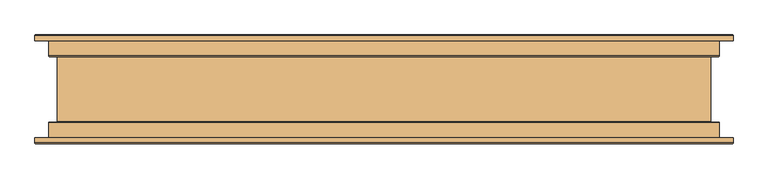
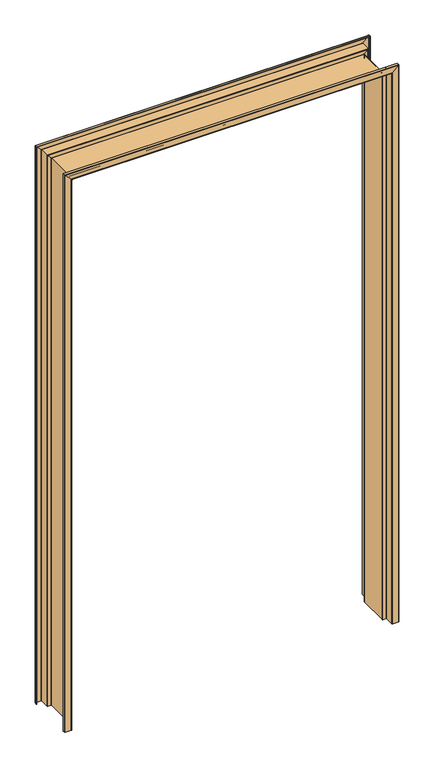
"""IFC4 building model written with IfcOpenShell, lengths in millimetres: door geometry, Porta Dupla de Abrir : 120x210cm - Marco Metálico."""

from ifc_helpers import new_model, si_unit, frame, origin, place, context, project, spatial, polyline, circle_curve, ellipse_curve, source, transform, mapped, element, save
from ifc_brep_helpers import plane_surface, cylinder_surface, revolved_surface, advanced_brep


def door_964c49d4(model_context):
    return source(origin(), model_context, "Body", "AdvancedBrep", [
        advanced_brep(
        [(-574.05, 57.1, 50.0), (-574.05, -57.1, 50.0), (-575.55, -58.6, 50.0), (-588.55, -58.6, 50.0), (-589.05, -59.1, 50.0), (-589.05, -94.1, 50.0), (-590.55, -95.6, 50.0), (-612.55, -95.6, 50.0), (-614.05, -94.1, 50.0), (-614.05, -85.6, 50.0), (-613.05, -85.6, 50.0), (-613.05, -94.1, 50.0), (-612.55, -94.6, 50.0), (-590.55, -94.6, 50.0), (-590.05, -94.1, 50.0), (-590.05, -59.1, 50.0), (-588.55, -57.6, 50.0), (-575.55, -57.6, 50.0), (-575.05, -57.1, 50.0), (-575.05, 57.1, 50.0), (-575.55, 57.6, 50.0), (-588.55, 57.6, 50.0), (-590.05, 59.1, 50.0), (-590.05, 94.1, 50.0), (-590.55, 94.6, 50.0), (-612.55, 94.6, 50.0), (-613.05, 94.1, 50.0), (-613.05, 85.6, 50.0), (-614.05, 85.6, 50.0), (-614.05, 94.1, 50.0), (-612.55, 95.6, 50.0), (-590.55, 95.6, 50.0), (-589.05, 94.1, 50.0), (-589.05, 59.1, 50.0), (-588.55, 58.6, 50.0), (-575.55, 58.6, 50.0), (-574.05, 57.1, 2174.05), (-574.05, -57.1, 2174.05), (-575.55, -58.6, 2175.55), (-588.55, -58.6, 2188.55), (-589.05, -59.1, 2189.05), (-589.05, -94.1, 2189.05), (-590.55, -95.6, 2190.55), (-612.55, -95.6, 2212.55), (-614.05, -94.1, 2214.05), (-614.05, -85.6, 2214.05), (-613.05, -85.6, 2213.05), (-613.05, -94.1, 2213.05), (-612.55, -94.6, 2212.55), (-590.55, -94.6, 2190.55), (-590.05, -94.1, 2190.05), (-590.05, -59.1, 2190.05), (-588.55, -57.6, 2188.55), (-575.55, -57.6, 2175.55), (-575.05, -57.1, 2175.05), (-575.05, 57.1, 2175.05), (-575.55, 57.6, 2175.55), (-588.55, 57.6, 2188.55), (-590.05, 59.1, 2190.05), (-590.05, 94.1, 2190.05), (-590.55, 94.6, 2190.55), (-612.55, 94.6, 2212.55), (-613.05, 94.1, 2213.05), (-613.05, 85.6, 2213.05), (-614.05, 85.6, 2214.05), (-614.05, 94.1, 2214.05), (-612.55, 95.6, 2212.55), (-590.55, 95.6, 2190.55), (-589.05, 94.1, 2189.05), (-589.05, 59.1, 2189.05), (-588.55, 58.6, 2188.55), (-575.55, 58.6, 2175.55), (574.05, 57.1, 50.0), (575.55, 58.6, 50.0), (588.55, 58.6, 50.0), (589.05, 59.1, 50.0), (589.05, 94.1, 50.0), (590.55, 95.6, 50.0), (612.55, 95.6, 50.0), (614.05, 94.1, 50.0), (614.05, 85.6, 50.0), (613.05, 85.6, 50.0), (613.05, 94.1, 50.0), (612.55, 94.6, 50.0), (590.55, 94.6, 50.0), (590.05, 94.1, 50.0), (590.05, 59.1, 50.0), (588.55, 57.6, 50.0), (575.55, 57.6, 50.0), (575.05, 57.1, 50.0), (575.05, -57.1, 50.0), (575.55, -57.6, 50.0), (588.55, -57.6, 50.0), (590.05, -59.1, 50.0), (590.05, -94.1, 50.0), (590.55, -94.6, 50.0), (612.55, -94.6, 50.0), (613.05, -94.1, 50.0), (613.05, -85.6, 50.0), (614.05, -85.6, 50.0), (614.05, -94.1, 50.0), (612.55, -95.6, 50.0), (590.55, -95.6, 50.0), (589.05, -94.1, 50.0), (589.05, -59.1, 50.0), (588.55, -58.6, 50.0), (575.55, -58.6, 50.0), (574.05, -57.1, 50.0), (574.05, 57.1, 2174.05), (575.55, 58.6, 2175.55), (588.55, 58.6, 2188.55), (589.05, 59.1, 2189.05), (589.05, 94.1, 2189.05), (590.55, 95.6, 2190.55), (612.55, 95.6, 2212.55), (614.05, 94.1, 2214.05), (614.05, 85.6, 2214.05), (613.05, 85.6, 2213.05), (613.05, 94.1, 2213.05), (612.55, 94.6, 2212.55), (590.55, 94.6, 2190.55), (590.05, 94.1, 2190.05), (590.05, 59.1, 2190.05), (588.55, 57.6, 2188.55), (575.55, 57.6, 2175.55), (575.05, 57.1, 2175.05), (575.05, -57.1, 2175.05), (575.55, -57.6, 2175.55), (588.55, -57.6, 2188.55), (590.05, -59.1, 2190.05), (590.05, -94.1, 2190.05), (590.55, -94.6, 2190.55), (612.55, -94.6, 2212.55), (613.05, -94.1, 2213.05), (613.05, -85.6, 2213.05), (614.05, -85.6, 2214.05), (614.05, -94.1, 2214.05), (612.55, -95.6, 2212.55), (590.55, -95.6, 2190.55), (589.05, -94.1, 2189.05), (589.05, -59.1, 2189.05), (588.55, -58.6, 2188.55), (575.55, -58.6, 2175.55), (574.05, -57.1, 2174.05)],
        [
            (0, 1),
            (1, 2, circle_curve(frame((-575.55, -57.1, 50.0), z_axis=(0.0, 0.0, -1.0), x_axis=(1.0, 0.0, 0.0)), 1.5)),
            (2, 3),
            (3, 4, circle_curve(frame((-588.55, -59.1, 50.0), z_axis=(0.0, 0.0, 1.0), x_axis=(1.0, 0.0, 0.0)), 0.5)),
            (4, 5),
            (5, 6, circle_curve(frame((-590.55, -94.1, 50.0), z_axis=(0.0, 0.0, -1.0), x_axis=(1.0, 0.0, 0.0)), 1.5)),
            (6, 7),
            (7, 8, circle_curve(frame((-612.55, -94.1, 50.0), z_axis=(0.0, 0.0, -1.0), x_axis=(1.0, 0.0, 0.0)), 1.5)),
            (8, 9),
            (9, 10),
            (10, 11),
            (11, 12, circle_curve(frame((-612.55, -94.1, 50.0), z_axis=(0.0, 0.0, 1.0), x_axis=(1.0, 0.0, 0.0)), 0.5)),
            (12, 13),
            (13, 14, circle_curve(frame((-590.55, -94.1, 50.0), z_axis=(0.0, 0.0, 1.0), x_axis=(1.0, 0.0, 0.0)), 0.5)),
            (14, 15),
            (15, 16, circle_curve(frame((-588.55, -59.1, 50.0), z_axis=(0.0, 0.0, -1.0), x_axis=(1.0, 0.0, 0.0)), 1.5)),
            (16, 17),
            (17, 18, circle_curve(frame((-575.55, -57.1, 50.0), z_axis=(0.0, 0.0, 1.0), x_axis=(1.0, 0.0, 0.0)), 0.5)),
            (18, 19),
            (19, 20, circle_curve(frame((-575.55, 57.1, 50.0), z_axis=(0.0, 0.0, 1.0), x_axis=(1.0, 0.0, 0.0)), 0.5)),
            (20, 21),
            (21, 22, circle_curve(frame((-588.55, 59.1, 50.0), z_axis=(0.0, 0.0, -1.0), x_axis=(1.0, 0.0, 0.0)), 1.5)),
            (22, 23),
            (23, 24, circle_curve(frame((-590.55, 94.1, 50.0), z_axis=(0.0, 0.0, 1.0), x_axis=(1.0, 0.0, 0.0)), 0.5)),
            (24, 25),
            (25, 26, circle_curve(frame((-612.55, 94.1, 50.0), z_axis=(0.0, 0.0, 1.0), x_axis=(1.0, 0.0, 0.0)), 0.5)),
            (26, 27),
            (27, 28),
            (28, 29),
            (29, 30, circle_curve(frame((-612.55, 94.1, 50.0), z_axis=(0.0, 0.0, -1.0), x_axis=(1.0, 0.0, 0.0)), 1.5)),
            (30, 31),
            (31, 32, circle_curve(frame((-590.55, 94.1, 50.0), z_axis=(0.0, 0.0, -1.0), x_axis=(1.0, 0.0, 0.0)), 1.5)),
            (32, 33),
            (33, 34, circle_curve(frame((-588.55, 59.1, 50.0), z_axis=(0.0, 0.0, 1.0), x_axis=(1.0, 0.0, 0.0)), 0.5)),
            (34, 35),
            (35, 0, circle_curve(frame((-575.55, 57.1, 50.0), z_axis=(0.0, 0.0, -1.0), x_axis=(1.0, 0.0, 0.0)), 1.5)),
            (0, 36),
            (36, 37),
            (37, 1),
            (37, 38, ellipse_curve(frame((-575.55, -57.1, 2175.55), z_axis=(-0.7071067811865475, 0.0, -0.7071067811865475), x_axis=(0.7071067811865474, 0.0, -0.7071067811865476)), 2.1213203, 1.5)),
            (38, 2),
            (38, 39),
            (39, 3),
            (39, 40, ellipse_curve(frame((-588.55, -59.1, 2188.55), z_axis=(0.7071067811865475, 0.0, 0.7071067811865475), x_axis=(-0.7071067811865474, 0.0, 0.7071067811865476)), 0.7071068, 0.5)),
            (40, 4),
            (40, 41),
            (41, 5),
            (41, 42, ellipse_curve(frame((-590.55, -94.1, 2190.55), z_axis=(-0.7071067811865475, 0.0, -0.7071067811865475), x_axis=(0.7071067811865474, 0.0, -0.7071067811865476)), 2.1213203, 1.5)),
            (42, 6),
            (42, 43),
            (43, 7),
            (43, 44, ellipse_curve(frame((-612.55, -94.1, 2212.55), z_axis=(-0.7071067811865475, 0.0, -0.7071067811865475), x_axis=(0.7071067811865474, 0.0, -0.7071067811865476)), 2.1213203, 1.5)),
            (44, 8),
            (44, 45),
            (45, 9),
            (45, 46),
            (46, 10),
            (46, 47),
            (47, 11),
            (47, 48, ellipse_curve(frame((-612.55, -94.1, 2212.55), z_axis=(0.7071067811865475, 0.0, 0.7071067811865475), x_axis=(-0.7071067811865474, 0.0, 0.7071067811865476)), 0.7071068, 0.5)),
            (48, 12),
            (48, 49),
            (49, 13),
            (49, 50, ellipse_curve(frame((-590.55, -94.1, 2190.55), z_axis=(0.7071067811865475, 0.0, 0.7071067811865475), x_axis=(-0.7071067811865474, 0.0, 0.7071067811865476)), 0.7071068, 0.5)),
            (50, 14),
            (50, 51),
            (51, 15),
            (51, 52, ellipse_curve(frame((-588.55, -59.1, 2188.55), z_axis=(-0.7071067811865475, 0.0, -0.7071067811865475), x_axis=(0.7071067811865474, 0.0, -0.7071067811865476)), 2.1213203, 1.5)),
            (52, 16),
            (52, 53),
            (53, 17),
            (53, 54, ellipse_curve(frame((-575.55, -57.1, 2175.55), z_axis=(0.7071067811865475, 0.0, 0.7071067811865475), x_axis=(-0.7071067811865474, 0.0, 0.7071067811865476)), 0.7071068, 0.5)),
            (54, 18),
            (54, 55),
            (55, 19),
            (55, 56, ellipse_curve(frame((-575.55, 57.1, 2175.55), z_axis=(0.7071067811865475, 0.0, 0.7071067811865475), x_axis=(-0.7071067811865474, 0.0, 0.7071067811865476)), 0.7071068, 0.5)),
            (56, 20),
            (56, 57),
            (57, 21),
            (57, 58, ellipse_curve(frame((-588.55, 59.1, 2188.55), z_axis=(-0.7071067811865475, 0.0, -0.7071067811865475), x_axis=(0.7071067811865474, 0.0, -0.7071067811865476)), 2.1213203, 1.5)),
            (58, 22),
            (58, 59),
            (59, 23),
            (59, 60, ellipse_curve(frame((-590.55, 94.1, 2190.55), z_axis=(0.7071067811865475, 0.0, 0.7071067811865475), x_axis=(-0.7071067811865474, 0.0, 0.7071067811865476)), 0.7071068, 0.5)),
            (60, 24),
            (60, 61),
            (61, 25),
            (61, 62, ellipse_curve(frame((-612.55, 94.1, 2212.55), z_axis=(0.7071067811865475, 0.0, 0.7071067811865475), x_axis=(-0.7071067811865474, 0.0, 0.7071067811865476)), 0.7071068, 0.5)),
            (62, 26),
            (62, 63),
            (63, 27),
            (63, 64),
            (64, 28),
            (64, 65),
            (65, 29),
            (65, 66, ellipse_curve(frame((-612.55, 94.1, 2212.55), z_axis=(-0.7071067811865475, 0.0, -0.7071067811865475), x_axis=(0.7071067811865474, 0.0, -0.7071067811865476)), 2.1213203, 1.5)),
            (66, 30),
            (66, 67),
            (67, 31),
            (67, 68, ellipse_curve(frame((-590.55, 94.1, 2190.55), z_axis=(-0.7071067811865475, 0.0, -0.7071067811865475), x_axis=(0.7071067811865474, 0.0, -0.7071067811865476)), 2.1213203, 1.5)),
            (68, 32),
            (68, 69),
            (69, 33),
            (69, 70, ellipse_curve(frame((-588.55, 59.1, 2188.55), z_axis=(0.7071067811865475, 0.0, 0.7071067811865475), x_axis=(-0.7071067811865474, 0.0, 0.7071067811865476)), 0.7071068, 0.5)),
            (70, 34),
            (70, 71),
            (71, 35),
            (71, 36, ellipse_curve(frame((-575.55, 57.1, 2175.55), z_axis=(-0.7071067811865475, 0.0, -0.7071067811865475), x_axis=(0.7071067811865474, 0.0, -0.7071067811865476)), 2.1213203, 1.5)),
            (72, 73, circle_curve(frame((575.55, 57.1, 50.0), z_axis=(0.0, 0.0, -1.0), x_axis=(-1.0, 0.0, 0.0)), 1.5)),
            (73, 74),
            (74, 75, circle_curve(frame((588.55, 59.1, 50.0), z_axis=(0.0, 0.0, 1.0), x_axis=(-1.0, 0.0, 0.0)), 0.5)),
            (75, 76),
            (76, 77, circle_curve(frame((590.55, 94.1, 50.0), z_axis=(0.0, 0.0, -1.0), x_axis=(-1.0, 0.0, 0.0)), 1.5)),
            (77, 78),
            (78, 79, circle_curve(frame((612.55, 94.1, 50.0), z_axis=(0.0, 0.0, -1.0), x_axis=(-1.0, 0.0, 0.0)), 1.5)),
            (79, 80),
            (80, 81),
            (81, 82),
            (82, 83, circle_curve(frame((612.55, 94.1, 50.0), z_axis=(0.0, 0.0, 1.0), x_axis=(-1.0, 0.0, 0.0)), 0.5)),
            (83, 84),
            (84, 85, circle_curve(frame((590.55, 94.1, 50.0), z_axis=(0.0, 0.0, 1.0), x_axis=(-1.0, 0.0, 0.0)), 0.5)),
            (85, 86),
            (86, 87, circle_curve(frame((588.55, 59.1, 50.0), z_axis=(0.0, 0.0, -1.0), x_axis=(-1.0, 0.0, 0.0)), 1.5)),
            (87, 88),
            (88, 89, circle_curve(frame((575.55, 57.1, 50.0), z_axis=(0.0, 0.0, 1.0), x_axis=(-1.0, 0.0, 0.0)), 0.5)),
            (89, 90),
            (90, 91, circle_curve(frame((575.55, -57.1, 50.0), z_axis=(0.0, 0.0, 1.0), x_axis=(-1.0, 0.0, 0.0)), 0.5)),
            (91, 92),
            (92, 93, circle_curve(frame((588.55, -59.1, 50.0), z_axis=(0.0, 0.0, -1.0), x_axis=(-1.0, 0.0, 0.0)), 1.5)),
            (93, 94),
            (94, 95, circle_curve(frame((590.55, -94.1, 50.0), z_axis=(0.0, 0.0, 1.0), x_axis=(-1.0, 0.0, 0.0)), 0.5)),
            (95, 96),
            (96, 97, circle_curve(frame((612.55, -94.1, 50.0), z_axis=(0.0, 0.0, 1.0), x_axis=(-1.0, 0.0, 0.0)), 0.5)),
            (97, 98),
            (98, 99),
            (99, 100),
            (100, 101, circle_curve(frame((612.55, -94.1, 50.0), z_axis=(0.0, 0.0, -1.0), x_axis=(-1.0, 0.0, 0.0)), 1.5)),
            (101, 102),
            (102, 103, circle_curve(frame((590.55, -94.1, 50.0), z_axis=(0.0, 0.0, -1.0), x_axis=(-1.0, 0.0, 0.0)), 1.5)),
            (103, 104),
            (104, 105, circle_curve(frame((588.55, -59.1, 50.0), z_axis=(0.0, 0.0, 1.0), x_axis=(-1.0, 0.0, 0.0)), 0.5)),
            (105, 106),
            (106, 107, circle_curve(frame((575.55, -57.1, 50.0), z_axis=(0.0, 0.0, -1.0), x_axis=(-1.0, 0.0, 0.0)), 1.5)),
            (107, 72),
            (108, 109, ellipse_curve(frame((575.55, 57.1, 2175.55), z_axis=(0.7071067811865475, 0.0, -0.7071067811865475), x_axis=(0.7071067811865474, 0.0, 0.7071067811865476)), 2.1213203, 1.5)),
            (109, 73),
            (72, 108),
            (109, 110),
            (110, 74),
            (110, 111, ellipse_curve(frame((588.55, 59.1, 2188.55), z_axis=(-0.7071067811865475, 0.0, 0.7071067811865475), x_axis=(-0.7071067811865474, 0.0, -0.7071067811865476)), 0.7071068, 0.5)),
            (111, 75),
            (111, 112),
            (112, 76),
            (112, 113, ellipse_curve(frame((590.55, 94.1, 2190.55), z_axis=(0.7071067811865475, 0.0, -0.7071067811865475), x_axis=(0.7071067811865474, 0.0, 0.7071067811865476)), 2.1213203, 1.5)),
            (113, 77),
            (113, 114),
            (114, 78),
            (114, 115, ellipse_curve(frame((612.55, 94.1, 2212.55), z_axis=(0.7071067811865475, 0.0, -0.7071067811865475), x_axis=(0.7071067811865474, 0.0, 0.7071067811865476)), 2.1213203, 1.5)),
            (115, 79),
            (115, 116),
            (116, 80),
            (116, 117),
            (117, 81),
            (117, 118),
            (118, 82),
            (118, 119, ellipse_curve(frame((612.55, 94.1, 2212.55), z_axis=(-0.7071067811865475, 0.0, 0.7071067811865475), x_axis=(-0.7071067811865474, 0.0, -0.7071067811865476)), 0.7071068, 0.5)),
            (119, 83),
            (119, 120),
            (120, 84),
            (120, 121, ellipse_curve(frame((590.55, 94.1, 2190.55), z_axis=(-0.7071067811865475, 0.0, 0.7071067811865475), x_axis=(-0.7071067811865474, 0.0, -0.7071067811865476)), 0.7071068, 0.5)),
            (121, 85),
            (121, 122),
            (122, 86),
            (122, 123, ellipse_curve(frame((588.55, 59.1, 2188.55), z_axis=(0.7071067811865475, 0.0, -0.7071067811865475), x_axis=(0.7071067811865474, 0.0, 0.7071067811865476)), 2.1213203, 1.5)),
            (123, 87),
            (123, 124),
            (124, 88),
            (124, 125, ellipse_curve(frame((575.55, 57.1, 2175.55), z_axis=(-0.7071067811865475, 0.0, 0.7071067811865475), x_axis=(-0.7071067811865474, 0.0, -0.7071067811865476)), 0.7071068, 0.5)),
            (125, 89),
            (125, 126),
            (126, 90),
            (126, 127, ellipse_curve(frame((575.55, -57.1, 2175.55), z_axis=(-0.7071067811865475, 0.0, 0.7071067811865475), x_axis=(-0.7071067811865474, 0.0, -0.7071067811865476)), 0.7071068, 0.5)),
            (127, 91),
            (127, 128),
            (128, 92),
            (128, 129, ellipse_curve(frame((588.55, -59.1, 2188.55), z_axis=(0.7071067811865475, 0.0, -0.7071067811865475), x_axis=(0.7071067811865474, 0.0, 0.7071067811865476)), 2.1213203, 1.5)),
            (129, 93),
            (129, 130),
            (130, 94),
            (130, 131, ellipse_curve(frame((590.55, -94.1, 2190.55), z_axis=(-0.7071067811865475, 0.0, 0.7071067811865475), x_axis=(-0.7071067811865474, 0.0, -0.7071067811865476)), 0.7071068, 0.5)),
            (131, 95),
            (131, 132),
            (132, 96),
            (132, 133, ellipse_curve(frame((612.55, -94.1, 2212.55), z_axis=(-0.7071067811865475, 0.0, 0.7071067811865475), x_axis=(-0.7071067811865474, 0.0, -0.7071067811865476)), 0.7071068, 0.5)),
            (133, 97),
            (133, 134),
            (134, 98),
            (134, 135),
            (135, 99),
            (135, 136),
            (136, 100),
            (136, 137, ellipse_curve(frame((612.55, -94.1, 2212.55), z_axis=(0.7071067811865475, 0.0, -0.7071067811865475), x_axis=(0.7071067811865474, 0.0, 0.7071067811865476)), 2.1213203, 1.5)),
            (137, 101),
            (137, 138),
            (138, 102),
            (138, 139, ellipse_curve(frame((590.55, -94.1, 2190.55), z_axis=(0.7071067811865475, 0.0, -0.7071067811865475), x_axis=(0.7071067811865474, 0.0, 0.7071067811865476)), 2.1213203, 1.5)),
            (139, 103),
            (139, 140),
            (140, 104),
            (140, 141, ellipse_curve(frame((588.55, -59.1, 2188.55), z_axis=(-0.7071067811865475, 0.0, 0.7071067811865475), x_axis=(-0.7071067811865474, 0.0, -0.7071067811865476)), 0.7071068, 0.5)),
            (141, 105),
            (141, 142),
            (142, 106),
            (142, 143, ellipse_curve(frame((575.55, -57.1, 2175.55), z_axis=(0.7071067811865475, 0.0, -0.7071067811865475), x_axis=(0.7071067811865474, 0.0, 0.7071067811865476)), 2.1213203, 1.5)),
            (143, 107),
            (143, 108),
            (36, 108),
            (143, 37),
            (142, 38),
            (141, 39),
            (140, 40),
            (139, 41),
            (138, 42),
            (137, 43),
            (136, 44),
            (135, 45),
            (134, 46),
            (133, 47),
            (132, 48),
            (131, 49),
            (130, 50),
            (129, 51),
            (128, 52),
            (127, 53),
            (126, 54),
            (125, 55),
            (124, 56),
            (123, 57),
            (122, 58),
            (121, 59),
            (120, 60),
            (119, 61),
            (118, 62),
            (117, 63),
            (116, 64),
            (115, 65),
            (114, 66),
            (113, 67),
            (112, 68),
            (111, 69),
            (110, 70),
            (109, 71),
        ],
        [
            plane_surface(frame((-600.0, -96.0340896, 50.0), z_axis=(0.0, 0.0, -1.0), x_axis=(1.0, 0.0, 0.0))),
            plane_surface(frame((-574.05, 57.1, 50.0), z_axis=(1.0, 0.0, 0.0), x_axis=(0.0, 0.0, 1.0))),
            cylinder_surface(frame((-575.55, -57.1, 50.0), z_axis=(0.0, 0.0, -1.0), x_axis=(1.0, 0.0, 0.0)), 1.5),
            plane_surface(frame((-575.55, -58.6, 50.0), z_axis=(0.0, -1.0, 0.0), x_axis=(0.0, 0.0, 1.0))),
            revolved_surface(polyline([(-588.05, -59.1, 2189.0500000133034), (-588.05, -59.1, 50.0)]), (-588.55, -59.1, 50.0), (0.0, 0.0, 1.0)),
            plane_surface(frame((-589.05, -59.1, 50.0), z_axis=(1.0, 0.0, 0.0), x_axis=(0.0, 0.0, 1.0))),
            cylinder_surface(frame((-590.55, -94.1, 50.0), z_axis=(0.0, 0.0, -1.0), x_axis=(1.0, 0.0, 0.0)), 1.5),
            plane_surface(frame((-590.55, -95.6, 50.0), z_axis=(0.0, -1.0, 0.0), x_axis=(0.0, 0.0, 1.0))),
            cylinder_surface(frame((-612.55, -94.1, 50.0), z_axis=(0.0, 0.0, -1.0), x_axis=(1.0, 0.0, 0.0)), 1.5),
            plane_surface(frame((-614.05, -94.1, 50.0), z_axis=(-1.0, 0.0, 0.0), x_axis=(0.0, 0.0, 1.0))),
            plane_surface(frame((-614.05, -85.6, 50.0), z_axis=(0.0, 1.0, 0.0), x_axis=(0.0, 0.0, 1.0))),
            plane_surface(frame((-613.05, -85.6, 50.0), z_axis=(1.0, 0.0, 0.0), x_axis=(0.0, 0.0, 1.0))),
            revolved_surface(polyline([(-612.05, -94.1, 2213.0500000133034), (-612.05, -94.1, 50.0)]), (-612.55, -94.1, 50.0), (0.0, 0.0, 1.0)),
            plane_surface(frame((-612.55, -94.6, 50.0), z_axis=(0.0, 1.0, 0.0), x_axis=(0.0, 0.0, 1.0))),
            revolved_surface(polyline([(-590.05, -94.1, 2191.0500000133034), (-590.05, -94.1, 50.0)]), (-590.55, -94.1, 50.0), (0.0, 0.0, 1.0)),
            plane_surface(frame((-590.05, -94.1, 50.0), z_axis=(-1.0, 0.0, 0.0), x_axis=(0.0, 0.0, 1.0))),
            cylinder_surface(frame((-588.55, -59.1, 50.0), z_axis=(0.0, 0.0, -1.0), x_axis=(1.0, 0.0, 0.0)), 1.5),
            plane_surface(frame((-588.55, -57.6, 50.0), z_axis=(0.0, 1.0, 0.0), x_axis=(0.0, 0.0, 1.0))),
            revolved_surface(polyline([(-575.05, -57.1, 2176.0500000133034), (-575.05, -57.1, 50.0)]), (-575.55, -57.1, 50.0), (0.0, 0.0, 1.0)),
            plane_surface(frame((-575.05, -57.1, 50.0), z_axis=(-1.0, 0.0, 0.0), x_axis=(0.0, 0.0, 1.0))),
            revolved_surface(polyline([(-575.05, 57.1, 2176.0500000133034), (-575.05, 57.1, 50.0)]), (-575.55, 57.1, 50.0), (0.0, 0.0, 1.0)),
            plane_surface(frame((-575.55, 57.6, 50.0), z_axis=(0.0, -1.0, 0.0), x_axis=(0.0, 0.0, 1.0))),
            cylinder_surface(frame((-588.55, 59.1, 50.0), z_axis=(0.0, 0.0, -1.0), x_axis=(1.0, 0.0, 0.0)), 1.5),
            plane_surface(frame((-590.05, 59.1, 50.0), z_axis=(-1.0, 0.0, 0.0), x_axis=(0.0, 0.0, 1.0))),
            revolved_surface(polyline([(-590.05, 94.1, 2191.0500000133034), (-590.05, 94.1, 50.0)]), (-590.55, 94.1, 50.0), (0.0, 0.0, 1.0)),
            plane_surface(frame((-590.55, 94.6, 50.0), z_axis=(0.0, -1.0, 0.0), x_axis=(0.0, 0.0, 1.0))),
            revolved_surface(polyline([(-612.05, 94.1, 2213.0500000133034), (-612.05, 94.1, 50.0)]), (-612.55, 94.1, 50.0), (0.0, 0.0, 1.0)),
            plane_surface(frame((-613.05, 94.1, 50.0), z_axis=(1.0, 0.0, 0.0), x_axis=(0.0, 0.0, 1.0))),
            plane_surface(frame((-613.05, 85.6, 50.0), z_axis=(0.0, -1.0, 0.0), x_axis=(0.0, 0.0, 1.0))),
            plane_surface(frame((-614.05, 85.6, 50.0), z_axis=(-1.0, 0.0, 0.0), x_axis=(0.0, 0.0, 1.0))),
            cylinder_surface(frame((-612.55, 94.1, 50.0), z_axis=(0.0, 0.0, -1.0), x_axis=(1.0, 0.0, 0.0)), 1.5),
            plane_surface(frame((-612.55, 95.6, 50.0), z_axis=(0.0, 1.0, 0.0), x_axis=(0.0, 0.0, 1.0))),
            cylinder_surface(frame((-590.55, 94.1, 50.0), z_axis=(0.0, 0.0, -1.0), x_axis=(1.0, 0.0, 0.0)), 1.5),
            plane_surface(frame((-589.05, 94.1, 50.0), z_axis=(1.0, 0.0, 0.0), x_axis=(0.0, 0.0, 1.0))),
            revolved_surface(polyline([(-588.05, 59.1, 2189.0500000133034), (-588.05, 59.1, 50.0)]), (-588.55, 59.1, 50.0), (0.0, 0.0, 1.0)),
            plane_surface(frame((-588.55, 58.6, 50.0), z_axis=(0.0, 1.0, 0.0), x_axis=(0.0, 0.0, 1.0))),
            cylinder_surface(frame((-575.55, 57.1, 50.0), z_axis=(0.0, 0.0, -1.0), x_axis=(1.0, 0.0, 0.0)), 1.5),
            plane_surface(frame((600.0, -96.0340896, 50.0), z_axis=(0.0, 0.0, -1.0), x_axis=(-1.0, 0.0, 0.0))),
            cylinder_surface(frame((575.55, 57.1, 2200.0), z_axis=(0.0, 0.0, 1.0), x_axis=(-1.0, 0.0, 0.0)), 1.5),
            plane_surface(frame((588.55, 58.6, 2188.55), z_axis=(0.0, 1.0, 0.0), x_axis=(0.0, 0.0, -1.0))),
            revolved_surface(polyline([(588.05, 59.1, 50.0), (588.05, 59.1, 2189.0500000133034)]), (588.55, 59.1, 2200.0), (0.0, 0.0, -1.0)),
            plane_surface(frame((589.05, 94.1, 2189.05), z_axis=(-1.0, 0.0, 0.0), x_axis=(0.0, 0.0, -1.0))),
            cylinder_surface(frame((590.55, 94.1, 2200.0), z_axis=(0.0, 0.0, 1.0), x_axis=(-1.0, 0.0, 0.0)), 1.5),
            plane_surface(frame((612.55, 95.6, 2212.55), z_axis=(0.0, 1.0, 0.0), x_axis=(0.0, 0.0, -1.0))),
            cylinder_surface(frame((612.55, 94.1, 2200.0), z_axis=(0.0, 0.0, 1.0), x_axis=(-1.0, 0.0, 0.0)), 1.5),
            plane_surface(frame((614.05, 85.6, 2214.05), z_axis=(1.0, 0.0, 0.0), x_axis=(0.0, 0.0, -1.0))),
            plane_surface(frame((613.05, 85.6, 2213.05), z_axis=(0.0, -1.0, 0.0), x_axis=(0.0, 0.0, -1.0))),
            plane_surface(frame((613.05, 94.1, 2213.05), z_axis=(-1.0, 0.0, 0.0), x_axis=(0.0, 0.0, -1.0))),
            revolved_surface(polyline([(612.05, 94.1, 50.0), (612.05, 94.1, 2213.0500000133034)]), (612.55, 94.1, 2200.0), (0.0, 0.0, -1.0)),
            plane_surface(frame((590.55, 94.6, 2190.55), z_axis=(0.0, -1.0, 0.0), x_axis=(0.0, 0.0, -1.0))),
            revolved_surface(polyline([(590.05, 94.1, 50.0), (590.05, 94.1, 2191.0500000133034)]), (590.55, 94.1, 2200.0), (0.0, 0.0, -1.0)),
            plane_surface(frame((590.05, 59.1, 2190.05), z_axis=(1.0, 0.0, 0.0), x_axis=(0.0, 0.0, -1.0))),
            cylinder_surface(frame((588.55, 59.1, 2200.0), z_axis=(0.0, 0.0, 1.0), x_axis=(-1.0, 0.0, 0.0)), 1.5),
            plane_surface(frame((575.55, 57.6, 2175.55), z_axis=(0.0, -1.0, 0.0), x_axis=(0.0, 0.0, -1.0))),
            revolved_surface(polyline([(575.05, 57.1, 50.0), (575.05, 57.1, 2176.0500000133034)]), (575.55, 57.1, 2200.0), (0.0, 0.0, -1.0)),
            plane_surface(frame((575.05, -57.1, 2175.05), z_axis=(1.0, 0.0, 0.0), x_axis=(0.0, 0.0, -1.0))),
            revolved_surface(polyline([(575.05, -57.1, 50.0), (575.05, -57.1, 2176.0500000133034)]), (575.55, -57.1, 2200.0), (0.0, 0.0, -1.0)),
            plane_surface(frame((588.55, -57.6, 2188.55), z_axis=(0.0, 1.0, 0.0), x_axis=(0.0, 0.0, -1.0))),
            cylinder_surface(frame((588.55, -59.1, 2200.0), z_axis=(0.0, 0.0, 1.0), x_axis=(-1.0, 0.0, 0.0)), 1.5),
            plane_surface(frame((590.05, -94.1, 2190.05), z_axis=(1.0, 0.0, 0.0), x_axis=(0.0, 0.0, -1.0))),
            revolved_surface(polyline([(590.05, -94.1, 50.0), (590.05, -94.1, 2191.0500000133034)]), (590.55, -94.1, 2200.0), (0.0, 0.0, -1.0)),
            plane_surface(frame((612.55, -94.6, 2212.55), z_axis=(0.0, 1.0, 0.0), x_axis=(0.0, 0.0, -1.0))),
            revolved_surface(polyline([(612.05, -94.1, 50.0), (612.05, -94.1, 2213.0500000133034)]), (612.55, -94.1, 2200.0), (0.0, 0.0, -1.0)),
            plane_surface(frame((613.05, -85.6, 2213.05), z_axis=(-1.0, 0.0, 0.0), x_axis=(0.0, 0.0, -1.0))),
            plane_surface(frame((614.05, -85.6, 2214.05), z_axis=(0.0, 1.0, 0.0), x_axis=(0.0, 0.0, -1.0))),
            plane_surface(frame((614.05, -94.1, 2214.05), z_axis=(1.0, 0.0, 0.0), x_axis=(0.0, 0.0, -1.0))),
            cylinder_surface(frame((612.55, -94.1, 2200.0), z_axis=(0.0, 0.0, 1.0), x_axis=(-1.0, 0.0, 0.0)), 1.5),
            plane_surface(frame((590.55, -95.6, 2190.55), z_axis=(0.0, -1.0, 0.0), x_axis=(0.0, 0.0, -1.0))),
            cylinder_surface(frame((590.55, -94.1, 2200.0), z_axis=(0.0, 0.0, 1.0), x_axis=(-1.0, 0.0, 0.0)), 1.5),
            plane_surface(frame((589.05, -59.1, 2189.05), z_axis=(-1.0, 0.0, 0.0), x_axis=(0.0, 0.0, -1.0))),
            revolved_surface(polyline([(588.05, -59.1, 50.0), (588.05, -59.1, 2189.0500000133034)]), (588.55, -59.1, 2200.0), (0.0, 0.0, -1.0)),
            plane_surface(frame((575.55, -58.6, 2175.55), z_axis=(0.0, -1.0, 0.0), x_axis=(0.0, 0.0, -1.0))),
            cylinder_surface(frame((575.55, -57.1, 2200.0), z_axis=(0.0, 0.0, 1.0), x_axis=(-1.0, 0.0, 0.0)), 1.5),
            plane_surface(frame((574.05, 57.1, 2174.05), z_axis=(-1.0, 0.0, 0.0), x_axis=(0.0, 0.0, -1.0))),
            plane_surface(frame((-574.05, 57.1, 2174.05), z_axis=(0.0, 0.0, -1.0), x_axis=(1.0, 0.0, 0.0))),
            cylinder_surface(frame((-600.0, -57.1, 2175.55), z_axis=(-1.0, 0.0, 0.0), x_axis=(0.0, 0.0, -1.0)), 1.5),
            plane_surface(frame((-575.55, -58.6, 2175.55), z_axis=(0.0, -1.0, 0.0), x_axis=(1.0, 0.0, 0.0))),
            revolved_surface(polyline([(589.0500000133031, -59.1, 2188.05), (-589.050000013303, -59.1, 2188.05)]), (-600.0, -59.1, 2188.55), (1.0, 0.0, 0.0)),
            plane_surface(frame((-589.05, -59.1, 2189.05), z_axis=(0.0, 0.0, -1.0), x_axis=(1.0, 0.0, 0.0))),
            cylinder_surface(frame((-600.0, -94.1, 2190.55), z_axis=(-1.0, 0.0, 0.0), x_axis=(0.0, 0.0, -1.0)), 1.5),
            plane_surface(frame((-590.55, -95.6, 2190.55), z_axis=(0.0, -1.0, 0.0), x_axis=(1.0, 0.0, 0.0))),
            cylinder_surface(frame((-600.0, -94.1, 2212.55), z_axis=(-1.0, 0.0, 0.0), x_axis=(0.0, 0.0, -1.0)), 1.5),
            plane_surface(frame((-614.05, -94.1, 2214.05), z_axis=(0.0, 0.0, 1.0), x_axis=(1.0, 0.0, 0.0))),
            plane_surface(frame((-614.05, -85.6, 2214.05), z_axis=(0.0, 1.0, 0.0), x_axis=(1.0, 0.0, 0.0))),
            plane_surface(frame((-613.05, -85.6, 2213.05), z_axis=(0.0, 0.0, -1.0), x_axis=(1.0, 0.0, 0.0))),
            revolved_surface(polyline([(613.0500000133031, -94.1, 2212.05), (-613.050000013303, -94.1, 2212.05)]), (-600.0, -94.1, 2212.55), (1.0, 0.0, 0.0)),
            plane_surface(frame((-612.55, -94.6, 2212.55), z_axis=(0.0, 1.0, 0.0), x_axis=(1.0, 0.0, 0.0))),
            revolved_surface(polyline([(591.0500000133031, -94.1, 2190.05), (-591.050000013303, -94.1, 2190.05)]), (-600.0, -94.1, 2190.55), (1.0, 0.0, 0.0)),
            plane_surface(frame((-590.05, -94.1, 2190.05), z_axis=(0.0, 0.0, 1.0), x_axis=(1.0, 0.0, 0.0))),
            cylinder_surface(frame((-600.0, -59.1, 2188.55), z_axis=(-1.0, 0.0, 0.0), x_axis=(0.0, 0.0, -1.0)), 1.5),
            plane_surface(frame((-588.55, -57.6, 2188.55), z_axis=(0.0, 1.0, 0.0), x_axis=(1.0, 0.0, 0.0))),
            revolved_surface(polyline([(576.0500000133031, -57.1, 2175.05), (-576.050000013303, -57.1, 2175.05)]), (-600.0, -57.1, 2175.55), (1.0, 0.0, 0.0)),
            plane_surface(frame((-575.05, -57.1, 2175.05), z_axis=(0.0, 0.0, 1.0), x_axis=(1.0, 0.0, 0.0))),
            revolved_surface(polyline([(576.0500000133031, 57.1, 2175.05), (-576.050000013303, 57.1, 2175.05)]), (-600.0, 57.1, 2175.55), (1.0, 0.0, 0.0)),
            plane_surface(frame((-575.55, 57.6, 2175.55), z_axis=(0.0, -1.0, 0.0), x_axis=(1.0, 0.0, 0.0))),
            cylinder_surface(frame((-600.0, 59.1, 2188.55), z_axis=(-1.0, 0.0, 0.0), x_axis=(0.0, 0.0, -1.0)), 1.5),
            plane_surface(frame((-590.05, 59.1, 2190.05), z_axis=(0.0, 0.0, 1.0), x_axis=(1.0, 0.0, 0.0))),
            revolved_surface(polyline([(591.0500000133031, 94.1, 2190.05), (-591.050000013303, 94.1, 2190.05)]), (-600.0, 94.1, 2190.55), (1.0, 0.0, 0.0)),
            plane_surface(frame((-590.55, 94.6, 2190.55), z_axis=(0.0, -1.0, 0.0), x_axis=(1.0, 0.0, 0.0))),
            revolved_surface(polyline([(613.0500000133031, 94.1, 2212.05), (-613.050000013303, 94.1, 2212.05)]), (-600.0, 94.1, 2212.55), (1.0, 0.0, 0.0)),
            plane_surface(frame((-613.05, 94.1, 2213.05), z_axis=(0.0, 0.0, -1.0), x_axis=(1.0, 0.0, 0.0))),
            plane_surface(frame((-613.05, 85.6, 2213.05), z_axis=(0.0, -1.0, 0.0), x_axis=(1.0, 0.0, 0.0))),
            plane_surface(frame((-614.05, 85.6, 2214.05), z_axis=(0.0, 0.0, 1.0), x_axis=(1.0, 0.0, 0.0))),
            cylinder_surface(frame((-600.0, 94.1, 2212.55), z_axis=(-1.0, 0.0, 0.0), x_axis=(0.0, 0.0, -1.0)), 1.5),
            plane_surface(frame((-612.55, 95.6, 2212.55), z_axis=(0.0, 1.0, 0.0), x_axis=(1.0, 0.0, 0.0))),
            cylinder_surface(frame((-600.0, 94.1, 2190.55), z_axis=(-1.0, 0.0, 0.0), x_axis=(0.0, 0.0, -1.0)), 1.5),
            plane_surface(frame((-589.05, 94.1, 2189.05), z_axis=(0.0, 0.0, -1.0), x_axis=(1.0, 0.0, 0.0))),
            revolved_surface(polyline([(589.0500000133031, 59.1, 2188.05), (-589.050000013303, 59.1, 2188.05)]), (-600.0, 59.1, 2188.55), (1.0, 0.0, 0.0)),
            plane_surface(frame((-588.55, 58.6, 2188.55), z_axis=(0.0, 1.0, 0.0), x_axis=(1.0, 0.0, 0.0))),
            cylinder_surface(frame((-600.0, 57.1, 2175.55), z_axis=(-1.0, 0.0, 0.0), x_axis=(0.0, 0.0, -1.0)), 1.5),
        ],
        [
            (0, [[1, 2, 3, 4, 5, 6, 7, 8, 9, 10, 11, 12, 13, 14, 15, 16, 17, 18, 19, 20, 21, 22, 23, 24, 25, 26, 27, 28, 29, 30, 31, 32, 33, 34, 35, 36]]),
            (1, [[-1, 37, 38, 39]]),
            (2, [[-2, -39, 40, 41]]),
            (3, [[-3, -41, 42, 43]]),
            (4, [[-4, -43, 44, 45]]),
            (5, [[-5, -45, 46, 47]]),
            (6, [[-6, -47, 48, 49]]),
            (7, [[-7, -49, 50, 51]]),
            (8, [[-8, -51, 52, 53]]),
            (9, [[-9, -53, 54, 55]]),
            (10, [[-10, -55, 56, 57]]),
            (11, [[-11, -57, 58, 59]]),
            (12, [[-12, -59, 60, 61]]),
            (13, [[-13, -61, 62, 63]]),
            (14, [[-14, -63, 64, 65]]),
            (15, [[-15, -65, 66, 67]]),
            (16, [[-16, -67, 68, 69]]),
            (17, [[-17, -69, 70, 71]]),
            (18, [[-18, -71, 72, 73]]),
            (19, [[-19, -73, 74, 75]]),
            (20, [[-20, -75, 76, 77]]),
            (21, [[-21, -77, 78, 79]]),
            (22, [[-22, -79, 80, 81]]),
            (23, [[-23, -81, 82, 83]]),
            (24, [[-24, -83, 84, 85]]),
            (25, [[-25, -85, 86, 87]]),
            (26, [[-26, -87, 88, 89]]),
            (27, [[-27, -89, 90, 91]]),
            (28, [[-28, -91, 92, 93]]),
            (29, [[-29, -93, 94, 95]]),
            (30, [[-30, -95, 96, 97]]),
            (31, [[-31, -97, 98, 99]]),
            (32, [[-32, -99, 100, 101]]),
            (33, [[-33, -101, 102, 103]]),
            (34, [[-34, -103, 104, 105]]),
            (35, [[-35, -105, 106, 107]]),
            (36, [[-36, -107, 108, -37]]),
            (37, [[109, 110, 111, 112, 113, 114, 115, 116, 117, 118, 119, 120, 121, 122, 123, 124, 125, 126, 127, 128, 129, 130, 131, 132, 133, 134, 135, 136, 137, 138, 139, 140, 141, 142, 143, 144]]),
            (38, [[145, 146, -109, 147]]),
            (39, [[148, 149, -110, -146]]),
            (40, [[150, 151, -111, -149]]),
            (41, [[152, 153, -112, -151]]),
            (42, [[154, 155, -113, -153]]),
            (43, [[156, 157, -114, -155]]),
            (44, [[158, 159, -115, -157]]),
            (45, [[160, 161, -116, -159]]),
            (46, [[162, 163, -117, -161]]),
            (47, [[164, 165, -118, -163]]),
            (48, [[166, 167, -119, -165]]),
            (49, [[168, 169, -120, -167]]),
            (50, [[170, 171, -121, -169]]),
            (51, [[172, 173, -122, -171]]),
            (52, [[174, 175, -123, -173]]),
            (53, [[176, 177, -124, -175]]),
            (54, [[178, 179, -125, -177]]),
            (55, [[180, 181, -126, -179]]),
            (56, [[182, 183, -127, -181]]),
            (57, [[184, 185, -128, -183]]),
            (58, [[186, 187, -129, -185]]),
            (59, [[188, 189, -130, -187]]),
            (60, [[190, 191, -131, -189]]),
            (61, [[192, 193, -132, -191]]),
            (62, [[194, 195, -133, -193]]),
            (63, [[196, 197, -134, -195]]),
            (64, [[198, 199, -135, -197]]),
            (65, [[200, 201, -136, -199]]),
            (66, [[202, 203, -137, -201]]),
            (67, [[204, 205, -138, -203]]),
            (68, [[206, 207, -139, -205]]),
            (69, [[208, 209, -140, -207]]),
            (70, [[210, 211, -141, -209]]),
            (71, [[212, 213, -142, -211]]),
            (72, [[214, 215, -143, -213]]),
            (73, [[216, -147, -144, -215]]),
            (74, [[-38, 217, -216, 218]]),
            (75, [[-40, -218, -214, 219]]),
            (76, [[-42, -219, -212, 220]]),
            (77, [[-44, -220, -210, 221]]),
            (78, [[-46, -221, -208, 222]]),
            (79, [[-48, -222, -206, 223]]),
            (80, [[-50, -223, -204, 224]]),
            (81, [[-52, -224, -202, 225]]),
            (82, [[-54, -225, -200, 226]]),
            (83, [[-56, -226, -198, 227]]),
            (84, [[-58, -227, -196, 228]]),
            (85, [[-60, -228, -194, 229]]),
            (86, [[-62, -229, -192, 230]]),
            (87, [[-64, -230, -190, 231]]),
            (88, [[-66, -231, -188, 232]]),
            (89, [[-68, -232, -186, 233]]),
            (90, [[-70, -233, -184, 234]]),
            (91, [[-72, -234, -182, 235]]),
            (92, [[-74, -235, -180, 236]]),
            (93, [[-76, -236, -178, 237]]),
            (94, [[-78, -237, -176, 238]]),
            (95, [[-80, -238, -174, 239]]),
            (96, [[-82, -239, -172, 240]]),
            (97, [[-84, -240, -170, 241]]),
            (98, [[-86, -241, -168, 242]]),
            (99, [[-88, -242, -166, 243]]),
            (100, [[-90, -243, -164, 244]]),
            (101, [[-92, -244, -162, 245]]),
            (102, [[-94, -245, -160, 246]]),
            (103, [[-96, -246, -158, 247]]),
            (104, [[-98, -247, -156, 248]]),
            (105, [[-100, -248, -154, 249]]),
            (106, [[-102, -249, -152, 250]]),
            (107, [[-104, -250, -150, 251]]),
            (108, [[-106, -251, -148, 252]]),
            (109, [[-108, -252, -145, -217]]),
        ],
    ),
    ])


if __name__ == "__main__":
    model = new_model("IFC4")
    model_context = context("Model", 3, world=origin())
    ifc_project = project(units=[si_unit("LENGTHUNIT", "METRE", prefix="MILLI")], contexts=[model_context])
    site = spatial("IfcSite", under=ifc_project)
    building = spatial("IfcBuilding", under=site)
    placement = place(None, origin())
    door_shape = door_964c49d4(model_context)
    element("IfcDoor", 1, ObjectType="Porta Dupla de Abrir : 120x210cm - Marco Metálico", at=placement, inside=building, context=model_context, shape_type="MappedRepresentation", body=[
        mapped(door_shape, transform((0.0, 0.0, 0.0), x_axis=(1.0, 0.0, 0.0), y_axis=(0.0, 1.0, 0.0), z_axis=(0.0, 0.0, 1.0))),
    ])
    save(model, "model.ifc")

# Revit data of these elements
# Type "Porta Dupla de Abrir : 120x210cm - Marco Metálico"
#   Type Mark = ""
#   SINAPI = ""
#   Maçaneta [instance default] = ""
#   Fechadura [instance default] = ""
#   Vão Luz (somente para informação) = 114.80 cm
#   Tolerância Folha Vertical = 0.30 cm
#   Módulo Básico M = 10.00 cm
#   Largura de Coordenação Modular Largura CM = 120.00 cm
#   Rough Width = 120.00 cm
#   Deslocamento da Horizontal da Folha = 1.00 cm
#   Altura de Coordenação Modular Largura CM = 220.00 cm
#   Rough Height = 220.00 cm
#   Altura Nominal = 212.40 cm
#   Ajuste de Coordenação Topo AC Topo = 0.00 cm
#   Ajuste de Coordenação Base AC Base = 5.00 cm
#   Ajuste de Coordenação AC = 0.00 cm
#   Tolerância Folha Horizontal = 0.20 cm
#   Largura Folha (somente para informação) = 58.70 cm
#   Espessura Folha = 3.50 cm
#   Maçaneta - Distância da Folha = 5.50 cm
#   Maçaneta - Altura = 100.00 cm
#   Largura Nominal (Largura Mn) = 117.80 cm
#   Distância do Nível = 0.30 cm
#   Aduela Interna Espessura = 1.10 cm
#   Aduela Externa Espessura = 2.60 cm
#   Altura Folha (somente para informação) = 211.90 cm
#   Height = 215.00 cm
#   Width = 120.00 cm
#   Número de Módulos Básicos nM Largura = 12
#   Número de Módulos Básicos nM Altura = 22
#   Marco Metálico = yes
#   Aduela de Madeira = no
#   Aduela Metálica de Canto = no
#   Guarnição Chanfrada = no
#   Batente - Material [instance default] = none
#   Painel - Material [instance default] = none
#   Construction Type = (empty or 0)
#   Model = ""
#   Function = (empty or 0)
#   Description = (empty or 0)
#   Wall Closure = (empty or 0)
#   Assembly Code = ""
# Element 1 (IfcDoor, "Porta Dupla de Abrir : 120x210cm - Marco Metálico")
#   Materials on its faces: "Porta - Maçaneta"
# Materials
#   "Porta - Maçaneta": class "Metal", colour RGB 189 187 185, transparency 0, Cost = 0
